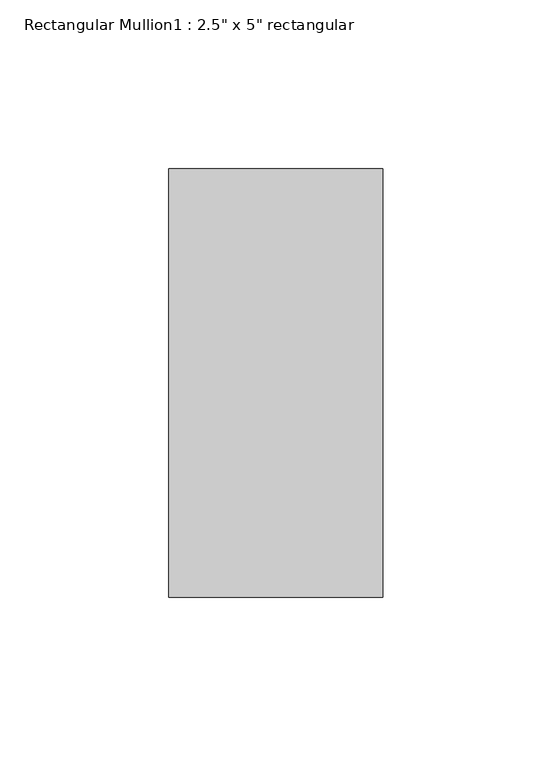
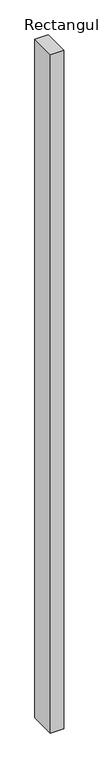
"""IFC4 building model written with IfcOpenShell, lengths in millimetres: member geometry."""

from ifc_helpers import new_model, si_unit, frame, origin, place, context, project, spatial, polyline, outline, extrude, source, transform, mapped, element, save


def member_349911e8(model_context):
    return source(origin(), model_context, "Body", "SweptSolid", [
        extrude(outline(polyline([(31.75, 63.5), (31.75, -63.5), (-31.75, -63.5), (-31.75, 63.5), (31.75, 63.5)])), frame((0.0, 0.0, -3414.1833333), z_axis=(0.0, 0.0, 1.0), x_axis=(1.0, 0.0, 0.0)), (0.0, 0.0, 1.0), 3414.1833333),
    ])


if __name__ == "__main__":
    model = new_model("IFC4")
    model_context = context("Model", 3, world=origin())
    ifc_project = project(units=[si_unit("LENGTHUNIT", "METRE", prefix="MILLI")], contexts=[model_context])
    site = spatial("IfcSite", under=ifc_project)
    building = spatial("IfcBuilding", under=site)
    placement = place(None, origin())
    member_shape = member_349911e8(model_context)
    element("IfcMember", 1, ObjectType="Rectangular Mullion1 : 2.5\" x 5\" rectangular", at=placement, inside=building, context=model_context, shape_type="MappedRepresentation", body=[
        mapped(member_shape, transform((0.0, 0.0, 0.0), x_axis=(1.0, 0.0, 0.0), y_axis=(0.0, 1.0, 0.0), z_axis=(0.0, 0.0, 1.0))),
    ])
    save(model, "model.ifc")

# Revit data of these elements
# Type "Rectangular Mullion1 : 2.5\" x 5\" rectangular"
#   built-in parameter 1007304 = 0.416667 (stored number, unit not read)
#   built-in parameter 1007301 = 0.104167 (stored number, unit not read)
#   built-in parameter 1007300 = 0.104167 (stored number, unit not read)
# Element 1 (IfcMember, "Rectangular Mullion1 : 2.5\" x 5\" rectangular")
#   Materials on its faces: "support-frame"
# Materials
#   "support-frame": class "Unassigned", colour RGB 233 233 233, transparency 0, Cost = 0
